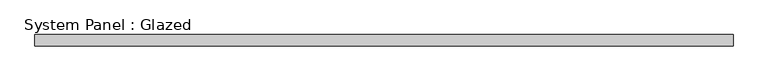
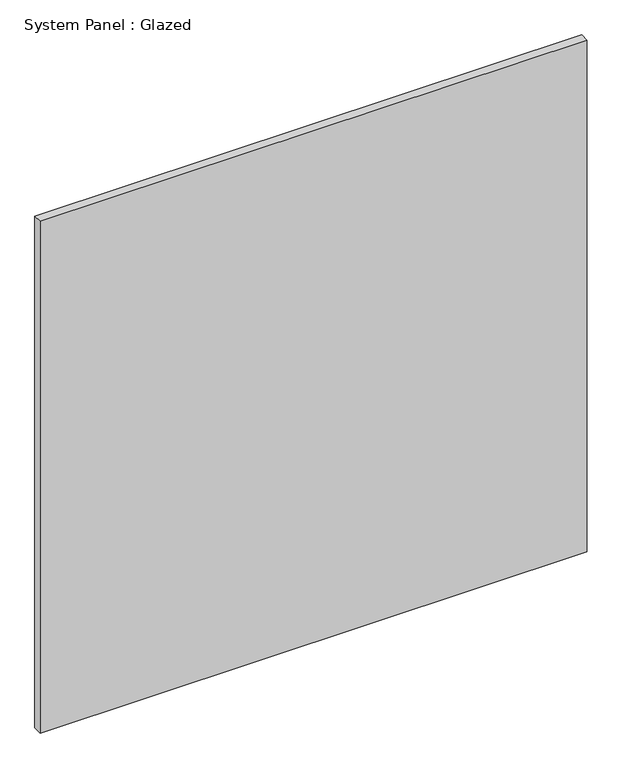
"""IFC4 building model written with IfcOpenShell, lengths in millimetres: plate geometry, System Panel : Glazed."""

from ifc_helpers import new_model, si_unit, origin, origin_with_axes, place, context, project, spatial, polyline, outline, extrude, source, transform, mapped, element, save


def system_panel_glazed_2613f10b(model_context):
    return source(origin(), model_context, "Body", "SweptSolid", [
        extrude(outline(polyline([(755.5084626, 24.5), (-755.5084626, 24.5), (-755.5084626, 49.5), (755.5084626, 49.5), (755.5084626, 24.5)])), origin_with_axes(), (0.0, 0.0, 1.0), 1494.0313026),
    ])


if __name__ == "__main__":
    model = new_model("IFC4")
    model_context = context("Model", 3, world=origin())
    ifc_project = project(units=[si_unit("LENGTHUNIT", "METRE", prefix="MILLI")], contexts=[model_context])
    site = spatial("IfcSite", under=ifc_project)
    building = spatial("IfcBuilding", under=site)
    placement = place(None, origin())
    system_panel_glazed_shape = system_panel_glazed_2613f10b(model_context)
    element("IfcPlate", 1, ObjectType="System Panel : Glazed", at=placement, inside=building, context=model_context, shape_type="MappedRepresentation", body=[
        mapped(system_panel_glazed_shape, transform((0.0, 0.0, 0.0), x_axis=(1.0, 0.0, 0.0), y_axis=(0.0, 1.0, 0.0), z_axis=(0.0, 0.0, 1.0))),
    ])
    save(model, "model.ifc")

# Revit data of these elements
# Element 1 (IfcPlate, "System Panel : Glazed")
#   Materials on its faces: "Glass"
# Materials
#   "Glass": class "Glass", colour RGB 218 227 224, transparency 0.85, Description = "Soda Lime Glass", Cost = 0
